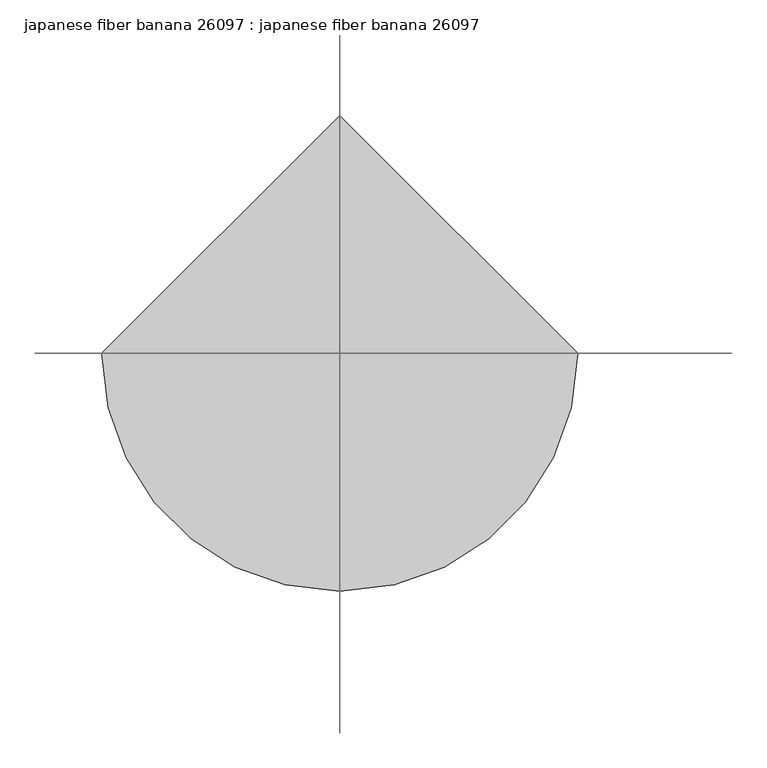
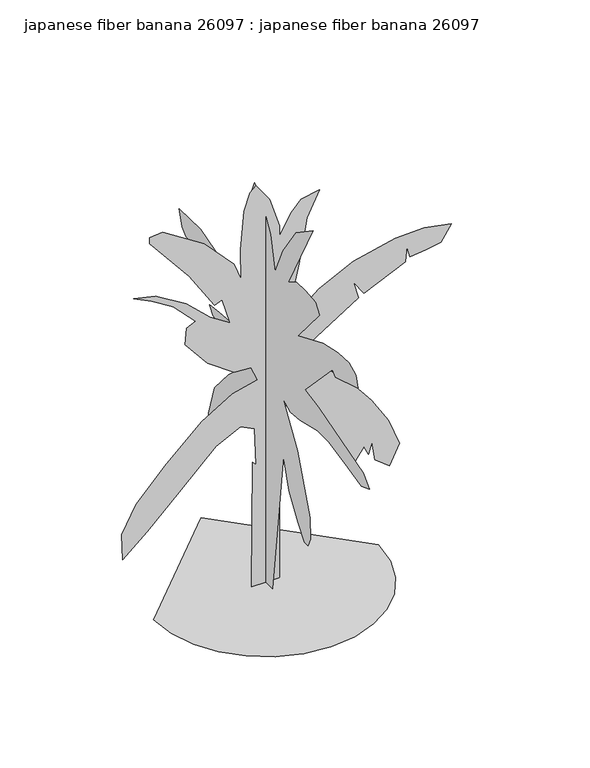
"""IFC4 building model written with IfcOpenShell, lengths in millimetres: proxy geometry, japanese fiber banana 26097 : japanese fiber banana 26097."""

import ifcopenshell
import ifcopenshell.guid

model = None  # the IFC model being written
_history = None  # IfcOwnerHistory: only IFC2X3 demands one
_inside = {}  # id of a spatial element -> (the spatial element, [elements in it])
_under = {}  # id of a project, library or spatial element -> (it, [spatial elements below it])
_declared = {}  # id of a project -> (the project, [libraries it declares])
_typed = {}  # id of a type object -> (the type object, [elements of that type])
_made_of = {}  # id of a material, layer set ... -> (it, [elements and type objects made of it])


def new_model(schema):
    """Start an empty IFC model of exactly this schema.

    Asked for "IFC4X3", IfcOpenShell would pick the latest addendum, in which some entities
    have other attributes; the version numbers below select the first issue.
    IFC2X3 requires an IfcOwnerHistory on every rooted entity: one is made here for all.
    """
    global model, _history
    if schema == "IFC4X3":
        model = ifcopenshell.file(schema_version=(4, 3, 0, 0))
    else:
        model = ifcopenshell.file(schema=schema)
    _inside.clear()
    _under.clear()
    _declared.clear()
    _typed.clear()
    _made_of.clear()
    _history = None
    if model.schema == "IFC2X3":
        org = make("IfcOrganization", Name="unknown")
        user = make(
            "IfcPersonAndOrganization",
            ThePerson=make("IfcPerson", FamilyName="unknown"),
            TheOrganization=org,
        )
        app = make(
            "IfcApplication",
            ApplicationDeveloper=org,
            Version="unknown",
            ApplicationFullName="unknown",
            ApplicationIdentifier="unknown",
        )
        _history = make(
            "IfcOwnerHistory",
            OwningUser=user,
            OwningApplication=app,
            ChangeAction="ADDED",
            CreationDate=0,
        )
    return model


def make(cls, **values):
    """One entity of the class cls with the attributes given. An attribute that is None is left unset."""
    return model.create_entity(
        cls, **{name: value for name, value in values.items() if value is not None}
    )


def rooted(cls, **values):
    """An entity with a GlobalId (a new one), such as an element, a storey or a relation."""
    return make(cls, GlobalId=ifcopenshell.guid.new(), OwnerHistory=_history, **values)


def si_unit(unit_type, name, prefix=None):
    """IfcSIUnit, for example si_unit("LENGTHUNIT", "METRE", prefix="MILLI")."""
    return make("IfcSIUnit", UnitType=unit_type, Prefix=prefix, Name=name)


def assignment(units):
    """IfcUnitAssignment: the units of a project."""
    return None if units is None else make("IfcUnitAssignment", Units=units)


def point(xyz):
    """IfcCartesianPoint."""
    return None if xyz is None else make("IfcCartesianPoint", Coordinates=xyz)


def direction(xyz):
    """IfcDirection."""
    return None if xyz is None else make("IfcDirection", DirectionRatios=xyz)


def frame(location, z_axis=None, x_axis=None):
    """IfcAxis2Placement3D, a coordinate frame: its origin and axes. An axis left out is left unset."""
    return make(
        "IfcAxis2Placement3D",
        Location=point(location),
        Axis=direction(z_axis),
        RefDirection=direction(x_axis),
    )


def origin():
    """The frame at (0, 0, 0) with its axes left unset."""
    return frame((0.0, 0.0, 0.0))


def place(relative_to, where):
    """IfcLocalPlacement: puts the frame where relative to a parent placement (None: the world)."""
    return make(
        "IfcLocalPlacement", PlacementRelTo=relative_to, RelativePlacement=where
    )


def context(
    kind, dimensions, precision=None, world=None, true_north=None, identifier=None
):
    """IfcGeometricRepresentationContext, for example the 3D "Model" context."""
    return make(
        "IfcGeometricRepresentationContext",
        ContextIdentifier=identifier,
        ContextType=kind,
        CoordinateSpaceDimension=dimensions,
        Precision=precision,
        WorldCoordinateSystem=world,
        TrueNorth=true_north,
    )


def project(units=None, contexts=None):
    """IfcProject with its units and contexts."""
    return rooted(
        "IfcProject",
        Name="project",
        RepresentationContexts=contexts,
        UnitsInContext=assignment(units),
    )


def spatial(cls, under=None, at=None, **own):
    """A site, building, storey or space (cls), placed at a placement, below another one or the project."""
    s = rooted(cls, ObjectPlacement=at, **own)
    if under is not None:
        _under.setdefault(under.id(), (under, []))[1].append(s)
    return s


def point_list(points):
    """IfcCartesianPointList2D or 3D."""
    cls = (
        "IfcCartesianPointList2D" if len(points[0]) == 2 else "IfcCartesianPointList3D"
    )
    return make(cls, CoordList=points)


def triangles(points, corners, closed=None, point_numbers=None):
    """IfcTriangulatedFaceSet: each triangle names its three corners, points numbered from 1."""
    return make(
        "IfcTriangulatedFaceSet",
        Coordinates=point_list(points),
        Closed=closed,
        CoordIndex=corners,
        PnIndex=point_numbers,
    )


def shape(context_of_items, identifier, shape_type, items):
    """IfcShapeRepresentation: the items that make up one representation, for example the "Body"."""
    return make(
        "IfcShapeRepresentation",
        ContextOfItems=context_of_items,
        RepresentationIdentifier=identifier,
        RepresentationType=shape_type,
        Items=items,
    )


def source(mapping_origin, context_of_items, identifier, shape_type, items):
    """IfcRepresentationMap: a shape defined once, which mapped items show again and again."""
    return make(
        "IfcRepresentationMap",
        MappingOrigin=mapping_origin,
        MappedRepresentation=shape(context_of_items, identifier, shape_type, items),
    )


def transform(
    local_origin,
    x_axis=None,
    y_axis=None,
    z_axis=None,
    scale=None,
    scale2=None,
    scale3=None,
    uniform=True,
):
    """IfcCartesianTransformationOperator3D, or its non-uniform kind. x_axis, y_axis, z_axis: its Axis1, 2, 3."""
    if uniform:
        return make(
            "IfcCartesianTransformationOperator3D",
            Axis1=direction(x_axis),
            Axis2=direction(y_axis),
            LocalOrigin=point(local_origin),
            Scale=scale,
            Axis3=direction(z_axis),
        )
    return make(
        "IfcCartesianTransformationOperator3DnonUniform",
        Axis1=direction(x_axis),
        Axis2=direction(y_axis),
        LocalOrigin=point(local_origin),
        Scale=scale,
        Axis3=direction(z_axis),
        Scale2=scale2,
        Scale3=scale3,
    )


def mapped(mapping_source, mapping_target):
    """IfcMappedItem: shows the shape of a source again, moved by a transform."""
    return make(
        "IfcMappedItem", MappingSource=mapping_source, MappingTarget=mapping_target
    )


def made_of(thing, what):
    """Note that an element or type object is made of a material, layer set ...; save() writes the relation."""
    if what is not None:
        _made_of.setdefault(what.id(), (what, []))[1].append(thing)
    return thing


def element(
    cls,
    number,
    at=None,
    inside=None,
    cuts=None,
    type_object=None,
    material=None,
    context=None,
    identifier="Body",
    shape_type=None,
    held_by="IfcProductDefinitionShape",
    body=None,
    shapes=None,
    **own,
):
    """One element of the class cls, such as IfcWall. Its Tag is "e" and its number.

    at: its placement. inside: the storey or other place that contains it. cuts: it is an
    opening in that element (IfcRelVoidsElement). A single representation is given by context,
    identifier, shape_type and body (its items); several are given by shapes. held_by: the class
    of the entity that holds the representations. save() writes the other relations.
    """
    e = rooted(cls, Tag="e%d" % number, ObjectPlacement=at, **own)
    if body is not None:
        shapes = [shape(context, identifier, shape_type, body)]
    if shapes is not None:
        e.Representation = make(held_by, Representations=shapes)
    if inside is not None:
        _inside.setdefault(inside.id(), (inside, []))[1].append(e)
    if cuts is not None:
        rooted(
            "IfcRelVoidsElement", RelatingBuildingElement=cuts, RelatedOpeningElement=e
        )
    if type_object is not None:
        _typed.setdefault(type_object.id(), (type_object, []))[1].append(e)
    return made_of(e, material)


def aggregate(whole, parts):
    """IfcRelAggregates: a whole, such as a stair, and the parts it consists of."""
    return rooted("IfcRelAggregates", RelatingObject=whole, RelatedObjects=parts)


def save(model, path):
    """Write the relations noted so far, then the file.

    IfcRelAggregates (storeys below a building ...), IfcRelContainedInSpatialStructure (elements
    in a storey), IfcRelDefinesByType, IfcRelAssociatesMaterial and IfcRelDeclares: one each for
    every whole, place, type object, material and project.
    """
    for whole, parts in _under.values():
        aggregate(whole, parts)
    for where, things in _inside.values():
        rooted(
            "IfcRelContainedInSpatialStructure",
            RelatedElements=things,
            RelatingStructure=where,
        )
    for kind, things in _typed.values():
        rooted("IfcRelDefinesByType", RelatedObjects=things, RelatingType=kind)
    for what, things in _made_of.values():
        rooted("IfcRelAssociatesMaterial", RelatedObjects=things, RelatingMaterial=what)
    for by, libraries in _declared.values():
        rooted("IfcRelDeclares", RelatingContext=by, RelatedDefinitions=libraries)
    model.write(path)


def japanese_fiber_banana_26097_japanese_fiber_banana_26097_fc2fb2a9(model_context):
    return source(origin(), model_context, "Body", "Tessellation", [
        triangles([(-649.7467501, 0.0, 3.7e-06), (-632.5712723, -148.8792756, 3.7e-06), (-583.6506755, -285.6010629, 3.7e-06), (-506.9043426, -406.2488949, 3.7e-06), (-406.2488949, -506.9043426, 3.7e-06), (-285.6010629, -583.6506755, 3.7e-06), (-148.8792756, -632.5712723, 3.7e-06), (2.84e-05, -649.7467501, 3.7e-06), (148.8792756, -632.5712723, 3.7e-06), (285.6010629, -583.6506755, 3.7e-06), (406.2488949, -506.9043426, 3.7e-06), (506.9043426, -406.2488949, 3.7e-06), (583.6506755, -285.6010629, 3.7e-06), (632.5712723, -148.8790212, 3.7e-06), (649.7467501, 5.68e-05, 3.7e-06), (-8.52e-05, 649.7467501, 3.7e-06), (73.5169788, -2.4e-06, 1488.9400761), (86.1999983, -4e-06, 1501.9626823), (108.3956093, -6.3e-06, 1521.7797867), (138.5178168, -9.4e-06, 1547.2586094), (174.9816703, -1.3e-05, 1577.2688416), (216.2016834, -1.69e-05, 1610.6750874), (260.5921424, -2.12e-05, 1646.3444218), (306.5688237, -2.56e-05, 1683.149152), (505.0933339, -3.74e-05, 1782.4125698), (746.7776007, -4.41e-05, 1838.5162674), (915.0912369, -4.46e-05, 1842.831847), (1070.4584976, -4.1e-05, 1812.6209003), (1010.0392931, -3.02e-05, 1721.9908218), (923.7222507, -2.81e-05, 1704.7264687), (833.0921722, -2.71e-05, 1696.0954548), (815.8277464, -3.48e-05, 1760.832637), (807.1968052, -2.45e-05, 1674.5181381), (565.5150455, -1.17e-05, 1566.6237064), (505.0933339, -2.2e-05, 1652.9382053), (535.3041716, -9.6e-06, 1549.3592079), (250.4636001, 1.15e-05, 1372.4146305), (207.3058056, 2.02e-05, 1299.0465797), (457.6205775, 4.54e-05, 1087.573078), (608.672295, 6.81e-05, 897.679509), (707.9358582, 8.66e-05, 742.3123209), (772.6704969, 0.0001061, 578.3115755), (712.2512924, 0.00012, 461.7861663), (630.2496843, 0.0001123, 526.5233485), (612.9878019, 9.89e-05, 638.7333235), (591.4078691, 0.0001066, 573.9961049), (565.5150455, 0.0001, 630.1023823), (518.0422892, 0.0001082, 561.0496931), (237.5161527, 6.86e-05, 893.3640747), (99.411601, 4.9e-05, 1057.362204), (82.1486921, 4.08e-05, 1126.4148932), (77.8327038, 0.0001751, 0.0), (-81.8504909, 0.0001751, 0.0), (-77.5347659, 8.45e-05, 759.5742033), (-55.9558732, 8.71e-05, 737.996814), (-64.587582, 6.09e-05, 958.1012569), (-146.5871735, 5.57e-05, 1001.2585064), (-289.0071958, 6.39e-05, 932.2058172), (-500.4806794, 8.86e-05, 725.0478951), (-686.0587051, 0.0001097, 548.1032813), (-828.4769743, 0.0001241, 427.259858), (-832.7950247, 0.0001056, 582.6295896), (-750.7934166, 8.71e-05, 737.996814), (-573.8488029, 6.5e-05, 923.574876), (-371.0062786, 4.28e-05, 1109.1529381), (-194.0604295, 3e-05, 1217.044899), (-47.3244142, 2.59e-05, 1251.5712799), (-86.1662158, 1.56e-05, 1337.8882496), (-185.4289796, 1.46e-05, 1346.5192635), (-336.4799704, 1.7e-06, 1454.4136951), (-465.9543348, -1.73e-05, 1614.0963902), (-457.3233936, -2.87e-05, 1709.0419029), (-405.5326232, -3.18e-05, 1734.93727), (-535.0069877, -4.77e-05, 1868.7272141), (-660.1633381, -5.7e-05, 1946.4106991), (-763.7423355, -6.31e-05, 1998.1989624), (-638.583478, -5.95e-05, 1967.9881611), (-461.6388642, -4.67e-05, 1860.0962002), (-323.5335222, -3.12e-05, 1730.6218357), (-207.0078768, -2.25e-05, 1657.2536396), (-254.4808694, -4.1e-05, 1812.6209003), (-297.6381552, -3.9e-05, 1795.3590179), (-444.3744384, -6.62e-05, 2024.0943295), (-673.1097862, -9.91e-05, 2300.30247), (-673.1097862, -0.0001038, 2339.1442852), (-595.4261559, -0.0001043, 2343.4597195), (-358.0598668, -8.63e-05, 2192.4080383), (-185.4289796, -6.42e-05, 2006.8299763), (-142.2711851, -5.13e-05, 1898.9380154), (-146.5871735, -7.29e-05, 2080.198027), (-125.0082762, -0.0001002, 2308.9359547), (-90.4819498, -0.000112, 2408.1969017), (-55.9558732, -0.0001156, 2438.4078484), (21.7278389, -0.0001027, 2330.5132713), (77.8327038, -8.11e-05, 2149.2507889), (77.8327038, -7.39e-05, 2088.8315117), (146.8851113, -8.78e-05, 2205.3569572), (202.9900806, -9.5e-05, 2265.7760891), (310.8842943, -9.76e-05, 2287.3560219), (237.5161527, -8.01e-05, 2140.619775), (190.0426515, -4.87e-05, 1877.3580826), (142.5693864, -2.3e-05, 1661.5692192), (124.24932, -1.81e-05, 1620.2990639), (106.9864112, -1.34e-05, 1581.1042179), (91.8370452, -9.2e-06, 1546.0623161), (79.8586157, -5.8e-06, 1517.2485226), (72.1077807, -3.4e-06, 1496.740472), (69.6416885, -2.1e-06, 1486.6108578), (-6.07e-05, -228.3904198, 1972.5652073), (-6.46e-05, -305.2429235, 2016.4820034), (-6.49e-05, -396.7365758, 2020.139629), (-6.39e-05, -495.5454429, 2009.1616653), (-5.9e-05, -535.8019973, 1954.2670509), (-3.61e-05, -319.883527, 1698.0893738), (-4.56e-05, -568.7408298, 1804.2211224), (-4.86e-05, -718.786722, 1837.1573387), (-4.89e-05, -828.5760235, 1840.8175804), (-4.63e-05, -901.771483, 1811.5388443), (-4.01e-05, -920.0697121, 1742.0061699), (-3.38e-05, -696.8283966, 1672.4708794), (-3.65e-05, -667.5522039, 1701.7496155), (-1.06e-05, -393.0764068, 1412.635722), (-8.3e-06, -524.8241063, 1387.0172276), (3.5e-06, -974.9643265, 1255.2694553), (8.7e-06, -1037.1792789, 1196.7146719), (1.13e-05, -956.6660975, 1167.4360085), (8.7e-06, -821.2583015, 1196.7146719), (5.1e-06, -623.6354805, 1236.971299), (5.1e-06, -517.5038046, 1236.971299), (8.7e-06, -341.8393816, 1196.7146719), (9.7e-06, -246.688885, 1185.7342375), (6.4e-06, -169.8356182, 1222.3306229), (2.67e-05, -316.2233943, 995.4317545), (5.65e-05, -440.6507558, 662.4010649), (6.79e-05, -447.9710575, 534.3135707), (7.28e-05, -422.3525631, 479.4163765), (7.28e-05, -385.756105, 479.4163765), (6.53e-05, -323.5411526, 563.5896907), (5.32e-05, -232.0500619, 698.9975229), (3.75e-05, -177.1549025, 874.6619459), (5.84e-05, -147.8774926, 640.4427395), (0.0001157, -67.36457, 3.7e-06), (0.0001157, 82.6820898, 3.7e-06), (9.61e-05, 82.6820898, 219.5804016), (0.0001026, 64.3836201, 146.3870222), (7.84e-05, 35.1062147, 417.2039675), (4.99e-05, 35.1062147, 735.593981), (2.38e-05, 79.0221933, 1028.3680435), (2.8e-05, 174.1739435, 980.7936945), (4.14e-05, 331.5396469, 830.7452225), (5.19e-05, 430.3510211, 713.6355829), (5.84e-05, 444.9891174, 640.4427395), (5.58e-05, 470.6076118, 669.7214029), (6.33e-05, 466.9474792, 585.5480887), (6.01e-05, 529.1624316, 622.1445105), (6.5e-05, 551.1207933, 567.2498597), (5.45e-05, 573.0791914, 684.3594629), (3.75e-05, 514.5243716, 874.6619459), (2.28e-05, 375.4563704, 1039.3484779), (6.1e-06, 170.5143013, 1225.9908646), (1.8e-06, 272.9848271, 1273.567757), (-1.1e-06, 393.7545994, 1306.5039734), (2e-07, 459.6297209, 1291.8659134), (-1.1e-06, 529.1624316, 1306.5039734), (-5e-06, 565.7588533, 1350.4207695), (-6.4e-06, 466.9474792, 1365.0588295), (-7.7e-06, 254.6866163, 1379.6968895), (-1.32e-05, 331.5396469, 1441.911842), (-2.5e-05, 514.5243716, 1573.6594688), (-2.96e-05, 730.4453854, 1624.896603), (-2.96e-05, 799.9781324, 1624.896603), (-3.29e-05, 840.2346869, 1661.4929157), (-4.1e-05, 869.5133503, 1752.9841335), (-4.14e-05, 653.5923729, 1756.6442299), (-3.58e-05, 441.3289484, 1694.4292774), (-3.02e-05, 283.9652797, 1632.214325), (-1.62e-05, 108.2998484, 1474.8480583), (-5.35e-05, 152.215827, 1892.0520985), (-8.06e-05, 185.15287, 2195.804052), (-9.63e-05, 111.9594906, 2371.468475), (-9.01e-05, 46.0854001, 2301.9356552), (-7.67e-05, -45.4067079, 2151.889872), (-5.87e-05, -89.322691, 1950.6068092), (-7.44e-05, -169.8356182, 2126.2712322), (-9.14e-05, -301.5827909, 2316.5737152), (-0.0001016, -469.9294556, 2430.0231857)], [[15, 16, 1], [14, 15, 1], [14, 1, 2], [13, 14, 2], [13, 2, 3], [13, 3, 4], [12, 13, 4], [11, 12, 4], [11, 4, 5], [11, 5, 6], [11, 6, 7], [11, 7, 8], [11, 8, 9], [11, 9, 10], [75, 76, 77], [45, 46, 47], [53, 54, 55], [60, 61, 62], [98, 99, 100], [97, 98, 100], [27, 28, 29], [27, 29, 30], [47, 48, 49], [60, 62, 63], [59, 60, 63], [59, 63, 64], [58, 59, 64], [58, 64, 65], [74, 75, 77], [74, 77, 78], [73, 74, 78], [73, 78, 79], [42, 43, 44], [42, 44, 45], [41, 42, 45], [92, 93, 94], [91, 92, 94], [96, 97, 100], [96, 100, 101], [52, 53, 55], [51, 52, 55], [51, 55, 56], [57, 58, 65], [57, 65, 66], [57, 66, 67], [27, 30, 31], [27, 31, 32], [26, 27, 32], [84, 85, 86], [83, 84, 86], [83, 86, 87], [83, 87, 88], [82, 83, 88], [81, 82, 88], [81, 88, 89], [56, 57, 67], [51, 56, 67], [91, 94, 95], [90, 91, 95], [90, 95, 96], [89, 90, 96], [89, 96, 101], [89, 101, 102], [33, 34, 35], [32, 33, 35], [26, 32, 35], [25, 26, 35], [24, 25, 35], [81, 89, 102], [80, 81, 102], [80, 102, 103], [80, 103, 104], [80, 104, 105], [80, 105, 106], [80, 106, 107], [40, 41, 45], [40, 45, 47], [40, 47, 49], [39, 40, 49], [38, 39, 49], [38, 49, 50], [38, 50, 51], [38, 51, 67], [38, 67, 68], [35, 36, 37], [24, 35, 37], [23, 24, 37], [22, 23, 37], [21, 22, 37], [20, 21, 37], [19, 20, 37], [18, 19, 37], [17, 18, 37], [17, 37, 38], [17, 38, 68], [108, 17, 68], [80, 107, 108], [80, 108, 68], [80, 68, 69], [80, 69, 70], [80, 70, 71], [79, 80, 71], [73, 79, 71], [73, 71, 72], [143, 144, 145], [185, 186, 109], [184, 185, 109], [155, 156, 157], [183, 184, 109], [151, 152, 153], [153, 154, 155], [164, 165, 166], [163, 164, 166], [124, 125, 126], [179, 180, 181], [172, 173, 174], [171, 172, 174], [170, 171, 174], [169, 170, 174], [169, 174, 175], [142, 143, 145], [141, 142, 145], [141, 145, 146], [141, 146, 147], [140, 141, 147], [140, 147, 148], [162, 163, 166], [162, 166, 167], [161, 162, 167], [179, 181, 182], [178, 179, 182], [178, 182, 183], [153, 155, 157], [153, 157, 158], [151, 153, 158], [150, 151, 158], [150, 158, 159], [149, 150, 159], [149, 159, 160], [148, 149, 160], [124, 126, 127], [123, 124, 127], [123, 127, 128], [123, 128, 129], [118, 119, 120], [117, 118, 120], [116, 117, 120], [116, 120, 121], [115, 116, 121], [115, 121, 122], [114, 115, 122], [168, 169, 175], [168, 175, 176], [168, 176, 177], [167, 168, 177], [177, 178, 183], [122, 123, 129], [122, 129, 130], [112, 113, 114], [111, 112, 114], [110, 111, 114], [109, 110, 114], [183, 109, 114], [177, 183, 114], [177, 114, 122], [177, 122, 130], [177, 130, 131], [177, 131, 132], [167, 177, 132], [161, 167, 132], [160, 161, 132], [148, 160, 132], [140, 148, 132], [140, 132, 133], [140, 133, 134], [139, 140, 134], [138, 139, 134], [138, 134, 135], [137, 138, 135], [137, 135, 136]], closed=False),
    ])


if __name__ == "__main__":
    model = new_model("IFC4")
    model_context = context("Model", 3, world=origin())
    ifc_project = project(units=[si_unit("LENGTHUNIT", "METRE", prefix="MILLI")], contexts=[model_context])
    site = spatial("IfcSite", under=ifc_project)
    building = spatial("IfcBuilding", under=site)
    placement = place(None, origin())
    japanese_fiber_banana_26097_japanese_fiber_banana_26097_shape = japanese_fiber_banana_26097_japanese_fiber_banana_26097_fc2fb2a9(model_context)
    element("IfcBuildingElementProxy", 1, Name="japanese fiber banana 26097 : japanese fiber banana 26097", ObjectType="japanese fiber banana 26097 : japanese fiber banana 26097", at=placement, inside=building, context=model_context, shape_type="MappedRepresentation", body=[
        mapped(japanese_fiber_banana_26097_japanese_fiber_banana_26097_shape, transform((0.0, 0.0, 0.0), x_axis=(1.0, 0.0, 0.0), y_axis=(0.0, 1.0, 0.0), z_axis=(0.0, 0.0, 1.0))),
    ])
    save(model, "model.ifc")

# Revit data of these elements
# Type "japanese fiber banana 26097 : japanese fiber banana 26097"
#   built-in parameter 1005195 = "RPC-16-FVGT-NR7X-7G1M-A000-ST1L-LVER-AU"
#   Height = 0
